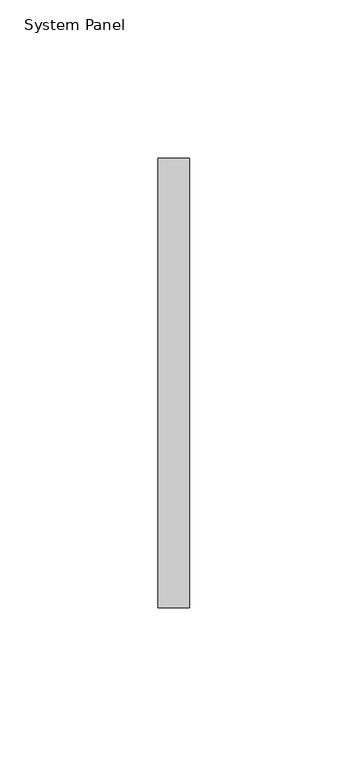
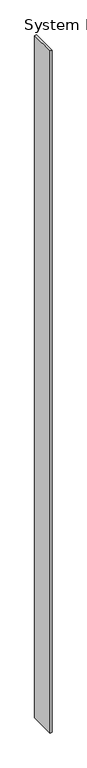
"""IFC4 building model written with IfcOpenShell, lengths in millimetres: plate geometry, System Panel : NLRS_21_CWP_hsb-vulling minerale wol 142 _gen_rsf."""

from ifc_helpers import new_model, si_unit, origin, origin_with_axes, place, context, project, spatial, polyline, outline, extrude, source, transform, mapped, element, save


def system_panel_1da55d1c(model_context):
    return source(origin(), model_context, "Body", "SweptSolid", [
        extrude(outline(polyline([(4.9999998, -71.0), (-4.9999998, -71.0), (-4.9999998, 71.0), (4.9999998, 71.0), (4.9999998, -71.0)])), origin_with_axes(), (0.0, 0.0, 1.0), 3849.0),
    ])


if __name__ == "__main__":
    model = new_model("IFC4")
    model_context = context("Model", 3, world=origin())
    ifc_project = project(units=[si_unit("LENGTHUNIT", "METRE", prefix="MILLI")], contexts=[model_context])
    site = spatial("IfcSite", under=ifc_project)
    building = spatial("IfcBuilding", under=site)
    placement = place(None, origin())
    system_panel_shape = system_panel_1da55d1c(model_context)
    element("IfcPlate", 1, ObjectType="System Panel : NLRS_21_CWP_hsb-vulling minerale wol 142 _gen_rsf", at=placement, inside=building, context=model_context, shape_type="MappedRepresentation", body=[
        mapped(system_panel_shape, transform((0.0, 0.0, 0.0), x_axis=(1.0, 0.0, 0.0), y_axis=(0.0, 1.0, 0.0), z_axis=(0.0, 0.0, 1.0))),
    ])
    save(model, "model.ifc")

# Revit data of these elements
# Type "System Panel : NLRS_21_CWP_hsb-vulling minerale wol 142 _gen_rsf"
#   Export Type to IFC As = "IfcWall"
#   Type IfcGUID = "07M7mRoiH1CR8m_RSKIwpC"
#   Assembly Code = "21.23"
# Element 1 (IfcPlate, "System Panel : NLRS_21_CWP_hsb-vulling minerale wol 142 _gen_rsf")
#   Materials on its faces: "NLRS_m1_isolatie minerale wol_gen_rsf"
# Materials
#   "NLRS_m1_isolatie minerale wol_gen_rsf": class "M - Anorganische materialen", colour RGB 200 200 140, transparency 0, Keynote = "m1", Manufacturer = "Revit Standards Foundation", URL = "www.revitstandards.org", Description = "isolatie minerale wol", Cost = 0
